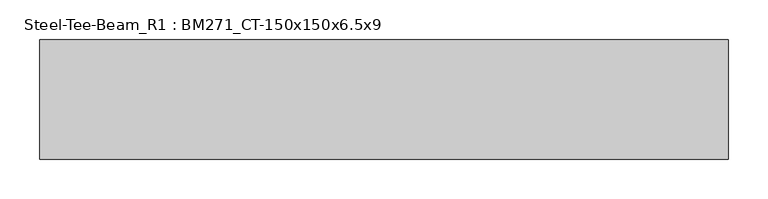
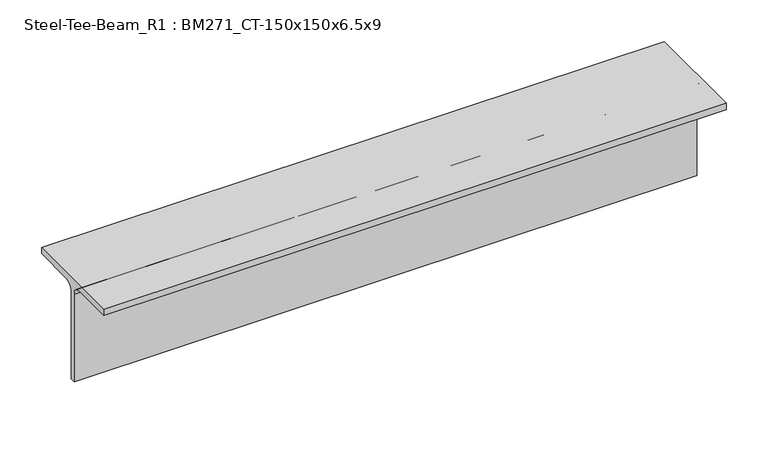
"""IFC4 building model written with IfcOpenShell, lengths in millimetres: member geometry, Steel-Tee-Beam_R1 : BM271_CT-150x150x6.5x9."""

from ifc_helpers import new_model, si_unit, point, frame, frame_2d, origin, place, context, project, spatial, polyline, circle_curve, trimmed, segment, composite_curve, outline, extrude, source, transform, mapped, element, save


def steel_tee_beam_r1_bm271_ct_150x150x6_5x9_a6d720bb(model_context):
    return source(origin(), model_context, "Body", "SweptSolid", [
        extrude(outline(composite_curve([segment(polyline([(75.0, 75.0), (75.0, 66.0), (16.25, 66.0)]), True, "CONTINUOUS"), segment(trimmed(circle_curve(frame_2d((16.25, 53.0)), 13.0), [point((16.25, 66.0))], [point((3.25, 53.0))], True, "CARTESIAN"), True, "CONTINUOUS"), segment(polyline([(3.25, 53.0), (3.25, -75.0), (-3.25, -75.0), (-3.25, 53.0)]), True, "CONTINUOUS"), segment(trimmed(circle_curve(frame_2d((-16.25, 53.0)), 13.0), [point((-3.25, 53.0))], [point((-16.25, 66.0))], True, "CARTESIAN"), True, "CONTINUOUS"), segment(polyline([(-16.25, 66.0), (-75.0, 66.0), (-75.0, 75.0), (75.0, 75.0)]), True, "CONTINUOUS")], self_intersect=False)), frame((-365.9474508, 0.0, 0.0), z_axis=(1.0, 0.0, 0.0), x_axis=(0.0, 1.0, 0.0)), (0.0, 0.0, 1.0), 865.9474508),
    ])


if __name__ == "__main__":
    model = new_model("IFC4")
    model_context = context("Model", 3, world=origin())
    ifc_project = project(units=[si_unit("LENGTHUNIT", "METRE", prefix="MILLI")], contexts=[model_context])
    site = spatial("IfcSite", under=ifc_project)
    building = spatial("IfcBuilding", under=site)
    placement = place(None, origin())
    steel_tee_beam_r1_bm271_ct_150x150x6_5x9_shape = steel_tee_beam_r1_bm271_ct_150x150x6_5x9_a6d720bb(model_context)
    element("IfcMember", 1, ObjectType="Steel-Tee-Beam_R1 : BM271_CT-150x150x6.5x9", at=placement, inside=building, context=model_context, shape_type="MappedRepresentation", body=[
        mapped(steel_tee_beam_r1_bm271_ct_150x150x6_5x9_shape, transform((0.0, 0.0, 0.0), x_axis=(1.0, 0.0, 0.0), y_axis=(0.0, 1.0, 0.0), z_axis=(0.0, 0.0, 1.0))),
    ])
    save(model, "model.ifc")

# Revit data of these elements
# Type "Steel-Tee-Beam_R1 : BM271_CT-150x150x6.5x9"
#   Keynote = "CT-150x150x6.5x9"
#   Surface Area = 0.588841 m²/m
#   Section Area = 23.3904 cm²
#   Mass per Unit Length = 18.3614 kg/m
#   Length [instance default] = 1.5240 m
#   bf = 0.1500 m
#   d = 0.1500 m
#   k = 0.0220 m
#   r = 0.0130 m
#   tf = 0.0090 m
#   tw = 0.0065 m
#   hec_material4 [instance default] = none
#   hec_material3 [instance default] = none
#   hec_material2 [instance default] = none
#   hec_material1 [instance default] = none
#   Structural Material [instance default] = Steel, 45-345
#   Assembly Code = ""
# Element 1 (IfcMember, "Steel-Tee-Beam_R1 : BM271_CT-150x150x6.5x9")
#   Structural Material = none
# Materials
#   "Steel, 45-345": class "Metal", colour RGB 189 187 185, transparency 0, Description = "Steel 345 MPa", Cost = 0
